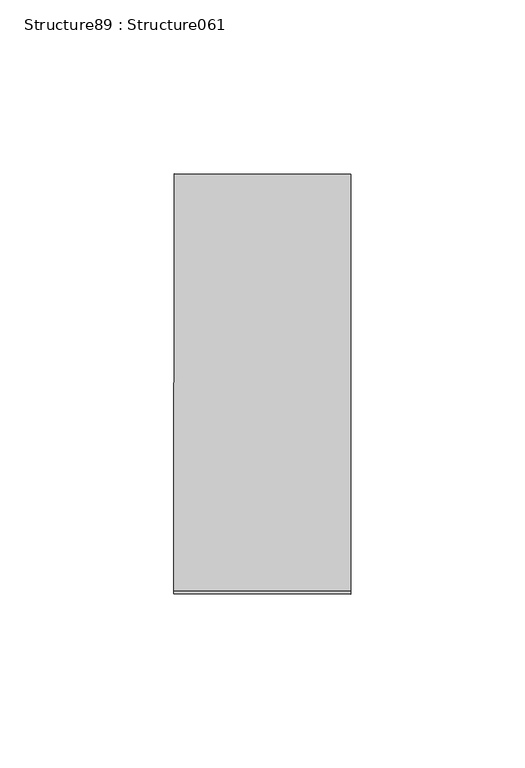
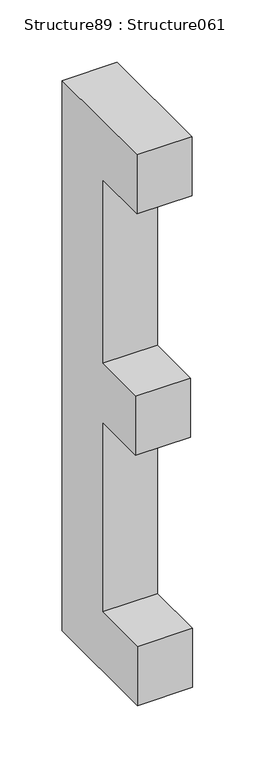
"""IFC4 building model written with IfcOpenShell, lengths in millimetres: proxy geometry, Structure89 : Structure061."""

import ifcopenshell
import ifcopenshell.guid

model = None  # the IFC model being written
_history = None  # IfcOwnerHistory: only IFC2X3 demands one
_inside = {}  # id of a spatial element -> (the spatial element, [elements in it])
_under = {}  # id of a project, library or spatial element -> (it, [spatial elements below it])
_declared = {}  # id of a project -> (the project, [libraries it declares])
_typed = {}  # id of a type object -> (the type object, [elements of that type])
_made_of = {}  # id of a material, layer set ... -> (it, [elements and type objects made of it])


def new_model(schema):
    """Start an empty IFC model of exactly this schema.

    Asked for "IFC4X3", IfcOpenShell would pick the latest addendum, in which some entities
    have other attributes; the version numbers below select the first issue.
    IFC2X3 requires an IfcOwnerHistory on every rooted entity: one is made here for all.
    """
    global model, _history
    if schema == "IFC4X3":
        model = ifcopenshell.file(schema_version=(4, 3, 0, 0))
    else:
        model = ifcopenshell.file(schema=schema)
    _inside.clear()
    _under.clear()
    _declared.clear()
    _typed.clear()
    _made_of.clear()
    _history = None
    if model.schema == "IFC2X3":
        org = make("IfcOrganization", Name="unknown")
        user = make(
            "IfcPersonAndOrganization",
            ThePerson=make("IfcPerson", FamilyName="unknown"),
            TheOrganization=org,
        )
        app = make(
            "IfcApplication",
            ApplicationDeveloper=org,
            Version="unknown",
            ApplicationFullName="unknown",
            ApplicationIdentifier="unknown",
        )
        _history = make(
            "IfcOwnerHistory",
            OwningUser=user,
            OwningApplication=app,
            ChangeAction="ADDED",
            CreationDate=0,
        )
    return model


def make(cls, **values):
    """One entity of the class cls with the attributes given. An attribute that is None is left unset."""
    return model.create_entity(
        cls, **{name: value for name, value in values.items() if value is not None}
    )


def rooted(cls, **values):
    """An entity with a GlobalId (a new one), such as an element, a storey or a relation."""
    return make(cls, GlobalId=ifcopenshell.guid.new(), OwnerHistory=_history, **values)


def si_unit(unit_type, name, prefix=None):
    """IfcSIUnit, for example si_unit("LENGTHUNIT", "METRE", prefix="MILLI")."""
    return make("IfcSIUnit", UnitType=unit_type, Prefix=prefix, Name=name)


def assignment(units):
    """IfcUnitAssignment: the units of a project."""
    return None if units is None else make("IfcUnitAssignment", Units=units)


def point(xyz):
    """IfcCartesianPoint."""
    return None if xyz is None else make("IfcCartesianPoint", Coordinates=xyz)


def direction(xyz):
    """IfcDirection."""
    return None if xyz is None else make("IfcDirection", DirectionRatios=xyz)


def frame(location, z_axis=None, x_axis=None):
    """IfcAxis2Placement3D, a coordinate frame: its origin and axes. An axis left out is left unset."""
    return make(
        "IfcAxis2Placement3D",
        Location=point(location),
        Axis=direction(z_axis),
        RefDirection=direction(x_axis),
    )


def origin():
    """The frame at (0, 0, 0) with its axes left unset."""
    return frame((0.0, 0.0, 0.0))


def place(relative_to, where):
    """IfcLocalPlacement: puts the frame where relative to a parent placement (None: the world)."""
    return make(
        "IfcLocalPlacement", PlacementRelTo=relative_to, RelativePlacement=where
    )


def context(
    kind, dimensions, precision=None, world=None, true_north=None, identifier=None
):
    """IfcGeometricRepresentationContext, for example the 3D "Model" context."""
    return make(
        "IfcGeometricRepresentationContext",
        ContextIdentifier=identifier,
        ContextType=kind,
        CoordinateSpaceDimension=dimensions,
        Precision=precision,
        WorldCoordinateSystem=world,
        TrueNorth=true_north,
    )


def project(units=None, contexts=None):
    """IfcProject with its units and contexts."""
    return rooted(
        "IfcProject",
        Name="project",
        RepresentationContexts=contexts,
        UnitsInContext=assignment(units),
    )


def spatial(cls, under=None, at=None, **own):
    """A site, building, storey or space (cls), placed at a placement, below another one or the project."""
    s = rooted(cls, ObjectPlacement=at, **own)
    if under is not None:
        _under.setdefault(under.id(), (under, []))[1].append(s)
    return s


def polyline(points):
    """IfcPolyline through the points."""
    return make("IfcPolyline", Points=[point(p) for p in points])


def outline(outer, holes=None, kind="AREA"):
    """IfcArbitraryClosedProfileDef: a profile drawn as a closed curve; with holes, ...WithVoids."""
    if holes is None:
        return make("IfcArbitraryClosedProfileDef", ProfileType=kind, OuterCurve=outer)
    return make(
        "IfcArbitraryProfileDefWithVoids",
        ProfileType=kind,
        OuterCurve=outer,
        InnerCurves=holes,
    )


def extrude(swept, where, along, depth):
    """IfcExtrudedAreaSolid: the profile swept, set in the frame where, extruded along a direction by depth."""
    return make(
        "IfcExtrudedAreaSolid",
        SweptArea=swept,
        Position=where,
        ExtrudedDirection=direction(along),
        Depth=depth,
    )


def shape(context_of_items, identifier, shape_type, items):
    """IfcShapeRepresentation: the items that make up one representation, for example the "Body"."""
    return make(
        "IfcShapeRepresentation",
        ContextOfItems=context_of_items,
        RepresentationIdentifier=identifier,
        RepresentationType=shape_type,
        Items=items,
    )


def source(mapping_origin, context_of_items, identifier, shape_type, items):
    """IfcRepresentationMap: a shape defined once, which mapped items show again and again."""
    return make(
        "IfcRepresentationMap",
        MappingOrigin=mapping_origin,
        MappedRepresentation=shape(context_of_items, identifier, shape_type, items),
    )


def transform(
    local_origin,
    x_axis=None,
    y_axis=None,
    z_axis=None,
    scale=None,
    scale2=None,
    scale3=None,
    uniform=True,
):
    """IfcCartesianTransformationOperator3D, or its non-uniform kind. x_axis, y_axis, z_axis: its Axis1, 2, 3."""
    if uniform:
        return make(
            "IfcCartesianTransformationOperator3D",
            Axis1=direction(x_axis),
            Axis2=direction(y_axis),
            LocalOrigin=point(local_origin),
            Scale=scale,
            Axis3=direction(z_axis),
        )
    return make(
        "IfcCartesianTransformationOperator3DnonUniform",
        Axis1=direction(x_axis),
        Axis2=direction(y_axis),
        LocalOrigin=point(local_origin),
        Scale=scale,
        Axis3=direction(z_axis),
        Scale2=scale2,
        Scale3=scale3,
    )


def mapped(mapping_source, mapping_target):
    """IfcMappedItem: shows the shape of a source again, moved by a transform."""
    return make(
        "IfcMappedItem", MappingSource=mapping_source, MappingTarget=mapping_target
    )


def made_of(thing, what):
    """Note that an element or type object is made of a material, layer set ...; save() writes the relation."""
    if what is not None:
        _made_of.setdefault(what.id(), (what, []))[1].append(thing)
    return thing


def element(
    cls,
    number,
    at=None,
    inside=None,
    cuts=None,
    type_object=None,
    material=None,
    context=None,
    identifier="Body",
    shape_type=None,
    held_by="IfcProductDefinitionShape",
    body=None,
    shapes=None,
    **own,
):
    """One element of the class cls, such as IfcWall. Its Tag is "e" and its number.

    at: its placement. inside: the storey or other place that contains it. cuts: it is an
    opening in that element (IfcRelVoidsElement). A single representation is given by context,
    identifier, shape_type and body (its items); several are given by shapes. held_by: the class
    of the entity that holds the representations. save() writes the other relations.
    """
    e = rooted(cls, Tag="e%d" % number, ObjectPlacement=at, **own)
    if body is not None:
        shapes = [shape(context, identifier, shape_type, body)]
    if shapes is not None:
        e.Representation = make(held_by, Representations=shapes)
    if inside is not None:
        _inside.setdefault(inside.id(), (inside, []))[1].append(e)
    if cuts is not None:
        rooted(
            "IfcRelVoidsElement", RelatingBuildingElement=cuts, RelatedOpeningElement=e
        )
    if type_object is not None:
        _typed.setdefault(type_object.id(), (type_object, []))[1].append(e)
    return made_of(e, material)


def aggregate(whole, parts):
    """IfcRelAggregates: a whole, such as a stair, and the parts it consists of."""
    return rooted("IfcRelAggregates", RelatingObject=whole, RelatedObjects=parts)


def save(model, path):
    """Write the relations noted so far, then the file.

    IfcRelAggregates (storeys below a building ...), IfcRelContainedInSpatialStructure (elements
    in a storey), IfcRelDefinesByType, IfcRelAssociatesMaterial and IfcRelDeclares: one each for
    every whole, place, type object, material and project.
    """
    for whole, parts in _under.values():
        aggregate(whole, parts)
    for where, things in _inside.values():
        rooted(
            "IfcRelContainedInSpatialStructure",
            RelatedElements=things,
            RelatingStructure=where,
        )
    for kind, things in _typed.values():
        rooted("IfcRelDefinesByType", RelatedObjects=things, RelatingType=kind)
    for what, things in _made_of.values():
        rooted("IfcRelAssociatesMaterial", RelatedObjects=things, RelatingMaterial=what)
    for by, libraries in _declared.values():
        rooted("IfcRelDeclares", RelatingContext=by, RelatedDefinitions=libraries)
    model.write(path)


def structure89_structure061_990c5e5f(model_context):
    return source(origin(), model_context, "Body", "SweptSolid", [
        extrude(outline(polyline([(537.7810299, 0.0), (537.7810299, -119.850495), (480.1634256, -119.850495), (480.1634256, -64.5410677), (300.3875053, -64.5410677), (300.3875053, -117.5426739), (242.7702568, -117.5426739), (242.7702568, -64.5410677), (57.6168926, -64.5410677), (57.6168926, -120.6165664), (0.0, -120.6165664), (0.0, 0.0), (537.7810299, 0.0)])), frame((-56111.7672021, 290737.7227783, -166.7961167), z_axis=(-0.9999998917542984, 0.00046528635450596156, 0.0), x_axis=(0.0, 0.0, 1.0)), (0.0, 0.0, 1.0), 50.8),
    ])


if __name__ == "__main__":
    model = new_model("IFC4")
    model_context = context("Model", 3, world=origin())
    ifc_project = project(units=[si_unit("LENGTHUNIT", "METRE", prefix="MILLI")], contexts=[model_context])
    site = spatial("IfcSite", under=ifc_project)
    building = spatial("IfcBuilding", under=site)
    placement = place(None, origin())
    structure89_structure061_shape = structure89_structure061_990c5e5f(model_context)
    element("IfcBuildingElementProxy", 1, Name="Structure89 : Structure061", ObjectType="Structure89 : Structure061", at=placement, inside=building, context=model_context, shape_type="MappedRepresentation", body=[
        mapped(structure89_structure061_shape, transform((0.0, 0.0, 0.0), x_axis=(1.0, 0.0, 0.0), y_axis=(0.0, 1.0, 0.0), z_axis=(0.0, 0.0, 1.0))),
    ])
    save(model, "model.ifc")

# Revit data of these elements
# Type "Structure89 : Structure061"
#   NameOverride = "Structure061"
# Element 1 (IfcBuildingElementProxy, "Structure89 : Structure061")
#   Materials on its faces: "BRUSHED ALUMINUM LETTERING"
# Materials
#   "BRUSHED ALUMINUM LETTERING": class "Unassigned", colour RGB 169 181 186, transparency 0, Cost = 0
